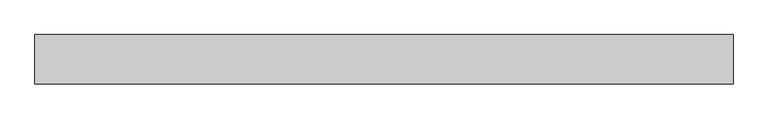
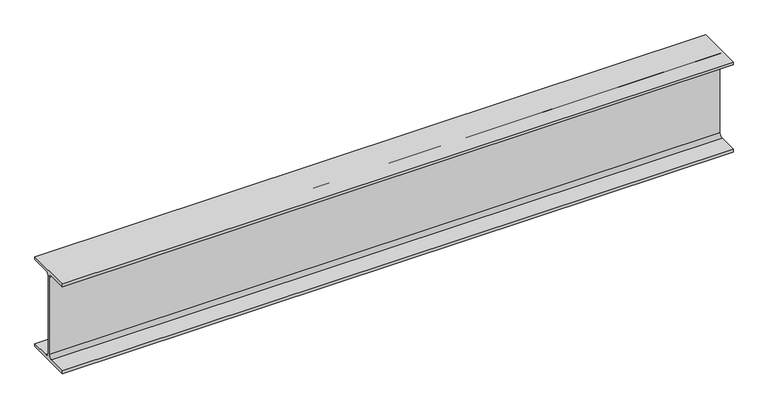
"""IFC4 building model written with IfcOpenShell, lengths in millimetres: beam geometry, 0912_Steel Framing_H-KSD3502 : H_SB_ASB_H-350x175x7x11."""

from ifc_helpers import new_model, si_unit, point, frame, frame_2d, origin, place, context, project, spatial, polyline, circle_curve, trimmed, segment, composite_curve, outline, extrude, source, transform, mapped, element, save


def beam_54b43205(model_context):
    return source(origin(), model_context, "Body", "SweptSolid", [
        extrude(outline(composite_curve([segment(polyline([(87.5, -164.0), (87.5, -175.0), (-87.5, -175.0), (-87.5, -164.0), (-17.5, -164.0)]), True, "CONTINUOUS"), segment(trimmed(circle_curve(frame_2d((-17.5, -150.0)), 14.0), [point((-17.5, -164.0))], [point((-3.5, -150.0))], True, "CARTESIAN"), True, "CONTINUOUS"), segment(polyline([(-3.5, -150.0), (-3.5, 150.0)]), True, "CONTINUOUS"), segment(trimmed(circle_curve(frame_2d((-17.5, 150.0)), 14.0), [point((-3.5, 150.0))], [point((-17.5, 164.0))], True, "CARTESIAN"), True, "CONTINUOUS"), segment(polyline([(-17.5, 164.0), (-87.5, 164.0), (-87.5, 175.0), (87.5, 175.0), (87.5, 164.0), (17.5, 164.0)]), True, "CONTINUOUS"), segment(trimmed(circle_curve(frame_2d((17.5, 150.0)), 14.0), [point((17.5, 164.0))], [point((3.5, 150.0))], True, "CARTESIAN"), True, "CONTINUOUS"), segment(polyline([(3.5, 150.0), (3.5, -150.0)]), True, "CONTINUOUS"), segment(trimmed(circle_curve(frame_2d((17.5, -150.0)), 14.0), [point((3.5, -150.0))], [point((17.5, -164.0))], True, "CARTESIAN"), True, "CONTINUOUS"), segment(polyline([(17.5, -164.0), (87.5, -164.0)]), True, "CONTINUOUS")], self_intersect=False)), frame((-1295.7739051, 0.0, 0.0), z_axis=(1.0, 0.0, 0.0), x_axis=(0.0, 1.0, 0.0)), (0.0, 0.0, 1.0), 2471.4118659),
    ])


if __name__ == "__main__":
    model = new_model("IFC4")
    model_context = context("Model", 3, world=origin())
    ifc_project = project(units=[si_unit("LENGTHUNIT", "METRE", prefix="MILLI")], contexts=[model_context])
    site = spatial("IfcSite", under=ifc_project)
    building = spatial("IfcBuilding", under=site)
    placement = place(None, origin())
    beam_shape = beam_54b43205(model_context)
    element("IfcBeam", 1, ObjectType="0912_Steel Framing_H-KSD3502 : H_SB_ASB_H-350x175x7x11", at=placement, inside=building, context=model_context, shape_type="MappedRepresentation", body=[
        mapped(beam_shape, transform((0.0, 0.0, 0.0), x_axis=(1.0, 0.0, 0.0), y_axis=(0.0, 1.0, 0.0), z_axis=(0.0, 0.0, 1.0))),
    ])
    save(model, "model.ifc")

# Revit data of these elements
# Type "0912_Steel Framing_H-KSD3502 : H_SB_ASB_H-350x175x7x11"
#   H_WM Code_1 = "S01AA002-00001 | Main Steel Structure Fabrication Work | Shelter/Building | Medium Steel - Standard (90KG/M>Weight≥30KG/M) | Material: (   )"
#   H_WM Code_2 = "S03AA028-00001 | Main Steel Structure Erection Work | Shelter/Building | Medium Steel (90KG/M>Weight≥30KG/M) | Material: (   )"
#   H_WM Code_3 = "S01AA010-00001 | Main Steel Structure Fabrication Work | Shelter/Building | Steel Painting/Coating | for Non-Fireproofed Steel Surface, Surface Preparation, Primer, Second & Final Coat | Material: (   )"
#   H_Q'ty Cal Type Tag = "SB-Q2"
#   Width = 17.5 cm
#   Web Thickness = 0.7 cm
#   Web Fillet = 1.4 cm
#   Warping Constant = 282000.0 cm⁶
#   W = 0
#   Torsional Moment of Inertia = 19.4042 cm⁴
#   Section Area = 63.14 cm²
#   Plastic Modulus weak axis = 174.0 cm³
#   Plastic Modulus strong axis = 868.0 cm³
#   Perimeter = 1.36 m²/m
#   Nominal Weight = 49.60 kgf/m
#   Moment of Inertia weak axis = 984.00 cm⁴
#   Moment of Inertia strong axis = 13600.00 cm⁴
#   Height = 35.0 cm
#   Flange Thickness = 1.1 cm
#   Elastic Modulus weak axis = 112.0 cm³
#   Elastic Modulus strong axis = 775.0 cm³
#   Centroid Vertical = 17.5 cm
#   Centroid Horizontal = 8.75 cm
#   Ix = 136000000
#   Length [instance default] = 1.5240 m
#   Zx = 868000
#   b = 0.1750 m
#   h = 0.3500 m
#   r = 0.0140 m
#   s = 0.0070 m
#   t = 0.0110 m
#   A = 0.006314 m²
#   Structural Material [instance default] = Steel, 45-345
#   Assembly Code = ""
# Element 1 (IfcBeam, "0912_Steel Framing_H-KSD3502 : H_SB_ASB_H-350x175x7x11")
#   Structural Material = none
# Materials
#   "Steel, 45-345": class "Metal", colour RGB 189 187 185, transparency 0, Description = "Steel 345 MPa", Cost = 0
